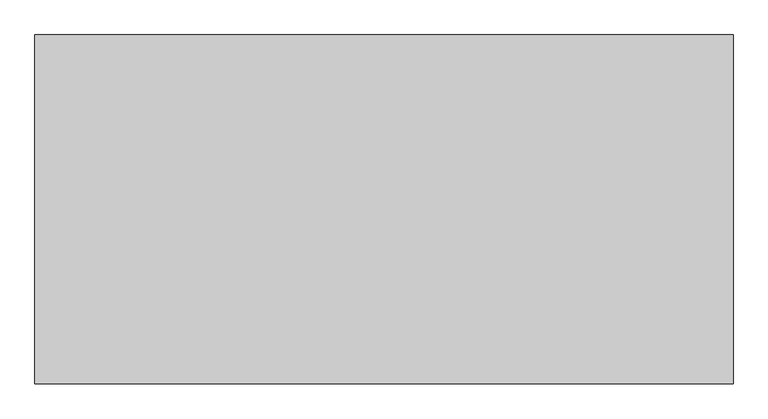
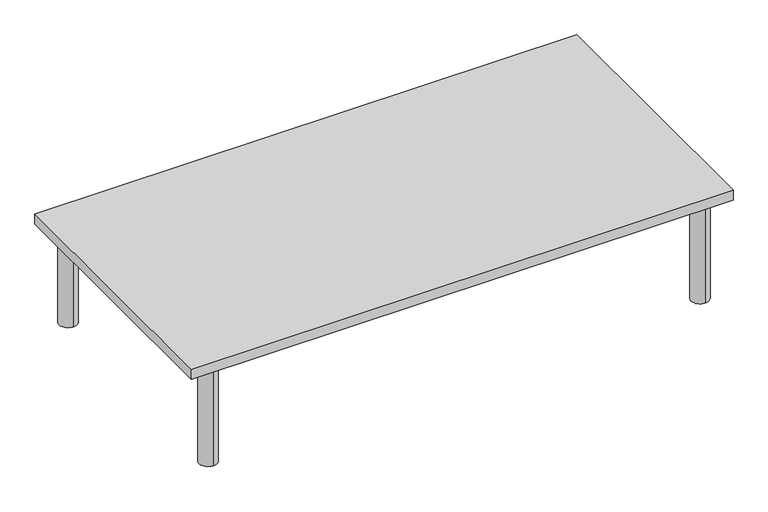
"""IFC4 building model written with IfcOpenShell, lengths in millimetres: furniture geometry, Table, Low-NON-COLLECTUS : -."""

from ifc_helpers import new_model, si_unit, point, frame, frame_2d, origin, origin_with_axes, place, context, project, spatial, polyline, circle_curve, trimmed, segment, composite_curve, outline, extrude, source, transform, mapped, element, save


def furniture_03aeb541(model_context):
    return source(origin(), model_context, "Body", "SweptSolid", [
        extrude(outline(composite_curve([segment(trimmed(circle_curve(frame_2d((-876.3, -431.8)), 31.75), [point((-876.3, -463.55))], [point((-876.3, -400.05))], False, "CARTESIAN"), True, "CONTINUOUS"), segment(trimmed(circle_curve(frame_2d((-876.3, -431.8)), 31.75), [point((-876.3, -400.05))], [point((-876.3, -463.55))], False, "CARTESIAN"), True, "CONTINUOUS")], self_intersect=False)), origin_with_axes(), (0.0, 0.0, 1.0), 368.3),
        extrude(outline(composite_curve([segment(trimmed(circle_curve(frame_2d((876.3, -431.8)), 31.75), [point((876.3, -463.55))], [point((876.3, -400.05))], False, "CARTESIAN"), True, "CONTINUOUS"), segment(trimmed(circle_curve(frame_2d((876.3, -431.8)), 31.75), [point((876.3, -400.05))], [point((876.3, -463.55))], False, "CARTESIAN"), True, "CONTINUOUS")], self_intersect=False)), origin_with_axes(), (0.0, 0.0, 1.0), 368.3),
        extrude(outline(polyline([(965.2, 482.6), (965.2, -482.6), (-965.2, -482.6), (-965.2, 482.6), (965.2, 482.6)])), frame((0.0, 0.0, 368.3), z_axis=(0.0, 0.0, 1.0), x_axis=(1.0, 0.0, 0.0)), (0.0, 0.0, 1.0), 38.1),
        extrude(outline(composite_curve([segment(trimmed(circle_curve(frame_2d((-876.3, 431.8)), 31.75), [point((-876.3, 463.55))], [point((-876.3, 400.05))], False, "CARTESIAN"), True, "CONTINUOUS"), segment(trimmed(circle_curve(frame_2d((-876.3, 431.8)), 31.75), [point((-876.3, 400.05))], [point((-876.3, 463.55))], False, "CARTESIAN"), True, "CONTINUOUS")], self_intersect=False)), origin_with_axes(), (0.0, 0.0, 1.0), 368.3),
        extrude(outline(composite_curve([segment(trimmed(circle_curve(frame_2d((876.3, 431.8)), 31.75), [point((876.3, 463.55))], [point((876.3, 400.05))], False, "CARTESIAN"), True, "CONTINUOUS"), segment(trimmed(circle_curve(frame_2d((876.3, 431.8)), 31.75), [point((876.3, 400.05))], [point((876.3, 463.55))], False, "CARTESIAN"), True, "CONTINUOUS")], self_intersect=False)), origin_with_axes(), (0.0, 0.0, 1.0), 368.3),
    ])


if __name__ == "__main__":
    model = new_model("IFC4")
    model_context = context("Model", 3, world=origin())
    ifc_project = project(units=[si_unit("LENGTHUNIT", "METRE", prefix="MILLI")], contexts=[model_context])
    site = spatial("IfcSite", under=ifc_project)
    building = spatial("IfcBuilding", under=site)
    placement = place(None, origin())
    furniture_shape = furniture_03aeb541(model_context)
    element("IfcFurniture", 1, ObjectType="Table, Low-NON-COLLECTUS : -", at=placement, inside=building, context=model_context, shape_type="MappedRepresentation", body=[
        mapped(furniture_shape, transform((0.0, 0.0, 0.0), x_axis=(1.0, 0.0, 0.0), y_axis=(0.0, 1.0, 0.0), z_axis=(0.0, 0.0, 1.0))),
    ])
    save(model, "model.ifc")

# Revit data of these elements
# Project information
#   Project Issue Date = "Issue Date"
#   Project Status = "Project Status"
#   Client Name = "Owner"
#   Project Address = "Enter address here"
#   Project Name = "Project Name"
#   Project Number = "0001"
# Type "Table, Low-NON-COLLECTUS : -"
#   External ID [instance default] = ""
#   Width = 1930.4 mm
#   Height = 406.4 mm
#   Depth = 965.2 mm
#   White = White
#   Default Elevation = 0
# Element 1 (IfcFurniture, "Table, Low-NON-COLLECTUS : -")
#   Materials on its faces: "White"
# Materials
#   "White": class "Generic", colour RGB 255 255 255, transparency 0, Cost = 0
